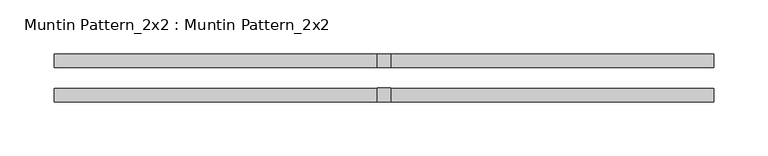
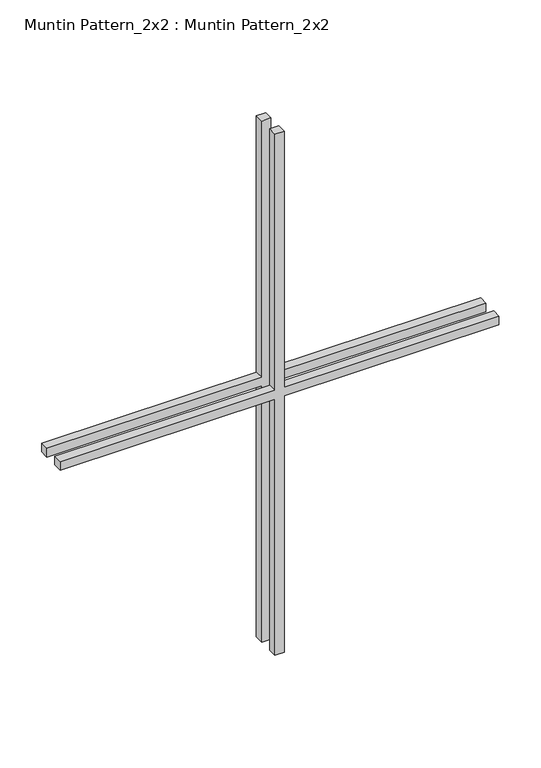
"""IFC4 building model written with IfcOpenShell, lengths in millimetres: proxy geometry, Muntin Pattern_2x2 : Muntin Pattern_2x2."""

from ifc_helpers import new_model, si_unit, frame, origin, place, context, project, spatial, polyline, outline, extrude, source, transform, mapped, element, save


def muntin_pattern_2x2_muntin_pattern_2x2_98ac56b0(model_context):
    return source(origin(), model_context, "Body", "SweptSolid", [
        extrude(outline(polyline([(388.9375, -6.35), (388.9375, -304.8), (376.2375, -304.8), (376.2375, -6.35), (0.0, -6.35), (0.0, 6.35), (376.2375, 6.35), (376.2375, 304.8), (388.9375, 304.8), (388.9375, 6.35), (765.175, 6.35), (765.175, -6.35), (388.9375, -6.35)])), frame((0.0, 9.525, 0.0), z_axis=(0.0, 1.0, 0.0), x_axis=(0.0, 0.0, 1.0)), (0.0, 0.0, 1.0), 12.7),
        extrude(outline(polyline([(388.9375, -6.35), (388.9375, -304.8), (376.2375, -304.8), (376.2375, -6.35), (0.0, -6.35), (0.0, 6.35), (376.2375, 6.35), (376.2375, 304.8), (388.9375, 304.8), (388.9375, 6.35), (765.175, 6.35), (765.175, -6.35), (388.9375, -6.35)])), frame((0.0, -22.225, 0.0), z_axis=(0.0, 1.0, 0.0), x_axis=(0.0, 0.0, 1.0)), (0.0, 0.0, 1.0), 12.7),
    ])


if __name__ == "__main__":
    model = new_model("IFC4")
    model_context = context("Model", 3, world=origin())
    ifc_project = project(units=[si_unit("LENGTHUNIT", "METRE", prefix="MILLI")], contexts=[model_context])
    site = spatial("IfcSite", under=ifc_project)
    building = spatial("IfcBuilding", under=site)
    placement = place(None, origin())
    muntin_pattern_2x2_muntin_pattern_2x2_shape = muntin_pattern_2x2_muntin_pattern_2x2_98ac56b0(model_context)
    element("IfcBuildingElementProxy", 1, Name="Muntin Pattern_2x2 : Muntin Pattern_2x2", ObjectType="Muntin Pattern_2x2 : Muntin Pattern_2x2", at=placement, inside=building, context=model_context, shape_type="MappedRepresentation", body=[
        mapped(muntin_pattern_2x2_muntin_pattern_2x2_shape, transform((0.0, 0.0, 0.0), x_axis=(1.0, 0.0, 0.0), y_axis=(0.0, 1.0, 0.0), z_axis=(0.0, 0.0, 1.0))),
    ])
    save(model, "model.ifc")

# Revit data of these elements
# Type "Muntin Pattern_2x2 : Muntin Pattern_2x2"
#   Width [instance default] = 4' - 0"
#   Thickness = 0' - 0 1/2"
#   Height [instance default] = 4' - 0"
#   Distance = 0' - 0 3/4"
#   Interior Material [instance default] = none
#   Exterior Material [instance default] = none
# Element 1 (IfcBuildingElementProxy, "Muntin Pattern_2x2 : Muntin Pattern_2x2")
#   Width = 2' - 0"
#   Height = 2' - 6 1/8"
#   Interior Material = 1X WOOD COMPOSITE TRIM
#   Exterior Material = 1X WOOD COMPOSITE TRIM
#   Materials on its faces: "1X WOOD COMPOSITE TRIM"
# Materials
#   "1X WOOD COMPOSITE TRIM": class "Generic", colour RGB 88 61 61, transparency 0, Cost = 0
